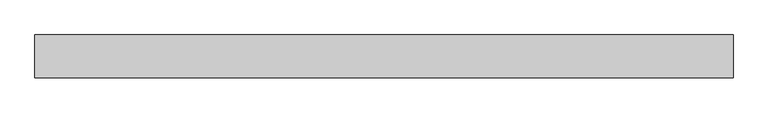
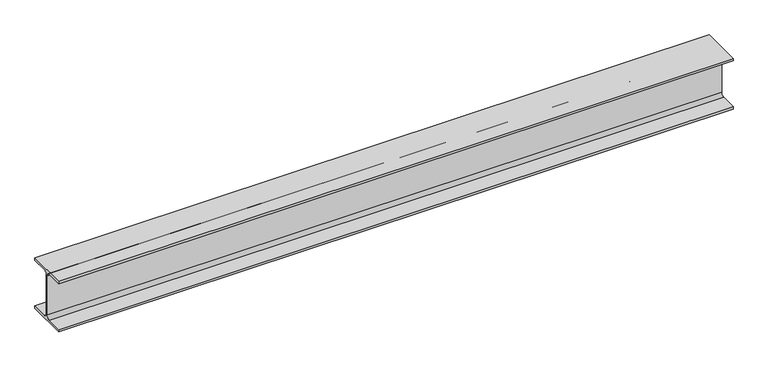
"""IFC4 building model written with IfcOpenShell, lengths in millimetres: beam geometry, 0912_Steel Framing_H-KSD3502 : H_SB_ASB_H-194x150x6x9."""

from ifc_helpers import new_model, si_unit, point, frame, frame_2d, origin, place, context, project, spatial, polyline, circle_curve, trimmed, segment, composite_curve, outline, extrude, source, transform, mapped, element, save


def beam_288211e0(model_context):
    return source(origin(), model_context, "Body", "SweptSolid", [
        extrude(outline(composite_curve([segment(polyline([(75.0, -88.0), (75.0, -97.0), (-75.0, -97.0), (-75.0, -88.0), (-16.0, -88.0)]), True, "CONTINUOUS"), segment(trimmed(circle_curve(frame_2d((-16.0, -75.0)), 13.0), [point((-16.0, -88.0))], [point((-3.0, -75.0))], True, "CARTESIAN"), True, "CONTINUOUS"), segment(polyline([(-3.0, -75.0), (-3.0, 75.0)]), True, "CONTINUOUS"), segment(trimmed(circle_curve(frame_2d((-16.0, 75.0)), 13.0), [point((-3.0, 75.0))], [point((-16.0, 88.0))], True, "CARTESIAN"), True, "CONTINUOUS"), segment(polyline([(-16.0, 88.0), (-75.0, 88.0), (-75.0, 97.0), (75.0, 97.0), (75.0, 88.0), (16.0, 88.0)]), True, "CONTINUOUS"), segment(trimmed(circle_curve(frame_2d((16.0, 75.0)), 13.0), [point((16.0, 88.0))], [point((3.0, 75.0))], True, "CARTESIAN"), True, "CONTINUOUS"), segment(polyline([(3.0, 75.0), (3.0, -75.0)]), True, "CONTINUOUS"), segment(trimmed(circle_curve(frame_2d((16.0, -75.0)), 13.0), [point((3.0, -75.0))], [point((16.0, -88.0))], True, "CARTESIAN"), True, "CONTINUOUS"), segment(polyline([(16.0, -88.0), (75.0, -88.0)]), True, "CONTINUOUS")], self_intersect=False)), frame((-1200.0, 0.0, 0.0), z_axis=(1.0, 0.0, 0.0), x_axis=(0.0, 1.0, 0.0)), (0.0, 0.0, 1.0), 2448.0465428),
    ])


if __name__ == "__main__":
    model = new_model("IFC4")
    model_context = context("Model", 3, world=origin())
    ifc_project = project(units=[si_unit("LENGTHUNIT", "METRE", prefix="MILLI")], contexts=[model_context])
    site = spatial("IfcSite", under=ifc_project)
    building = spatial("IfcBuilding", under=site)
    placement = place(None, origin())
    beam_shape = beam_288211e0(model_context)
    element("IfcBeam", 1, ObjectType="0912_Steel Framing_H-KSD3502 : H_SB_ASB_H-194x150x6x9", at=placement, inside=building, context=model_context, shape_type="MappedRepresentation", body=[
        mapped(beam_shape, transform((0.0, 0.0, 0.0), x_axis=(1.0, 0.0, 0.0), y_axis=(0.0, 1.0, 0.0), z_axis=(0.0, 0.0, 1.0))),
    ])
    save(model, "model.ifc")

# Revit data of these elements
# Type "0912_Steel Framing_H-KSD3502 : H_SB_ASB_H-194x150x6x9"
#   H_WM Code_1 = "S01AA002-00001 | Main Steel Structure Fabrication Work | Shelter/Building | Medium Steel - Standard (90KG/M>Weight≥30KG/M) | Material: (   )"
#   H_WM Code_2 = "S03AA028-00001 | Main Steel Structure Erection Work | Shelter/Building | Medium Steel (90KG/M>Weight≥30KG/M) | Material: (   )"
#   H_WM Code_3 = "S01AA010-00001 | Main Steel Structure Fabrication Work | Shelter/Building | Steel Painting/Coating | for Non-Fireproofed Steel Surface, Surface Preparation, Primer, Second & Final Coat | Material: (   )"
#   H_Q'ty Cal Type Tag = "SB-Q2"
#   Width = 15.0 cm
#   Web Thickness = 0.6 cm
#   Web Fillet = 1.3 cm
#   Warping Constant = 43316.0 cm⁶
#   W = 0
#   Torsional Moment of Inertia = 8.622 cm⁴
#   Section Area = 39.01 cm²
#   Plastic Modulus weak axis = 104.0 cm³
#   Plastic Modulus strong axis = 309.0 cm³
#   Perimeter = 0.95 m²/m
#   Nominal Weight = 30.60 kgf/m
#   Moment of Inertia weak axis = 507.00 cm⁴
#   Moment of Inertia strong axis = 2690.00 cm⁴
#   Height = 19.4 cm
#   Flange Thickness = 0.9 cm
#   Elastic Modulus weak axis = 67.6 cm³
#   Elastic Modulus strong axis = 277.0 cm³
#   Centroid Vertical = 9.7 cm
#   Centroid Horizontal = 7.5 cm
#   Ix = 26900000
#   Length [instance default] = 1.5240 m
#   Zx = 309000
#   b = 0.1500 m
#   h = 0.1940 m
#   r = 0.0130 m
#   s = 0.0060 m
#   t = 0.0090 m
#   A = 0.003901 m²
#   Structural Material [instance default] = Steel, 45-345
#   Assembly Code = ""
# Element 1 (IfcBeam, "0912_Steel Framing_H-KSD3502 : H_SB_ASB_H-194x150x6x9")
#   Structural Material = none
# Materials
#   "Steel, 45-345": class "Metal", colour RGB 189 187 185, transparency 0, Description = "Steel 345 MPa", Cost = 0
